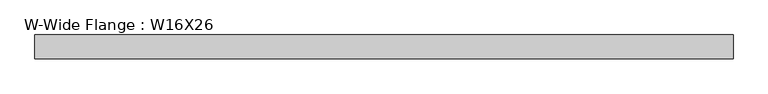
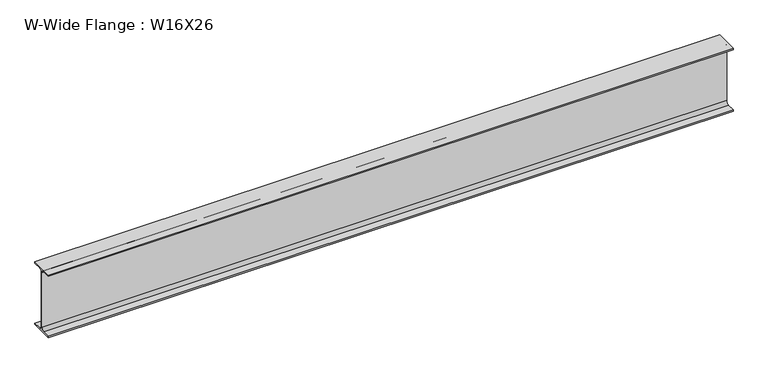
"""IFC4 building model written with IfcOpenShell, lengths in millimetres: beam geometry, W-Wide Flange : W16X26."""

from ifc_helpers import new_model, si_unit, point, frame, frame_2d, origin, place, context, project, spatial, polyline, circle_curve, trimmed, segment, composite_curve, outline, extrude, source, transform, mapped, element, save


def w_wide_flange_w16x26_55ea5116(model_context):
    return source(origin(), model_context, "Body", "SweptSolid", [
        extrude(outline(composite_curve([segment(polyline([(69.85, -190.627), (69.85, -199.39), (-69.85, -199.39), (-69.85, -190.627), (-21.3995, -190.627)]), True, "CONTINUOUS"), segment(trimmed(circle_curve(frame_2d((-21.3995, -172.4025)), 18.2245), [point((-21.3995, -190.627))], [point((-3.175, -172.4025))], True, "CARTESIAN"), True, "CONTINUOUS"), segment(polyline([(-3.175, -172.4025), (-3.175, 172.4025)]), True, "CONTINUOUS"), segment(trimmed(circle_curve(frame_2d((-21.3995, 172.4025)), 18.2245), [point((-3.175, 172.4025))], [point((-21.3995, 190.627))], True, "CARTESIAN"), True, "CONTINUOUS"), segment(polyline([(-21.3995, 190.627), (-69.85, 190.627), (-69.85, 199.39), (69.85, 199.39), (69.85, 190.627), (21.3995, 190.627)]), True, "CONTINUOUS"), segment(trimmed(circle_curve(frame_2d((21.3995, 172.4025)), 18.2245), [point((21.3995, 190.627))], [point((3.175, 172.4025))], True, "CARTESIAN"), True, "CONTINUOUS"), segment(polyline([(3.175, 172.4025), (3.175, -172.4025)]), True, "CONTINUOUS"), segment(trimmed(circle_curve(frame_2d((21.3995, -172.4025)), 18.2245), [point((3.175, -172.4025))], [point((21.3995, -190.627))], True, "CARTESIAN"), True, "CONTINUOUS"), segment(polyline([(21.3995, -190.627), (69.85, -190.627)]), True, "CONTINUOUS")], self_intersect=False)), frame((-2032.0, 0.0, 0.0), z_axis=(1.0, 0.0, 0.0), x_axis=(0.0, 1.0, 0.0)), (0.0, 0.0, 1.0), 4114.8),
    ])


if __name__ == "__main__":
    model = new_model("IFC4")
    model_context = context("Model", 3, world=origin())
    ifc_project = project(units=[si_unit("LENGTHUNIT", "METRE", prefix="MILLI")], contexts=[model_context])
    site = spatial("IfcSite", under=ifc_project)
    building = spatial("IfcBuilding", under=site)
    placement = place(None, origin())
    w_wide_flange_w16x26_shape = w_wide_flange_w16x26_55ea5116(model_context)
    element("IfcBeam", 1, ObjectType="W-Wide Flange : W16X26", at=placement, inside=building, context=model_context, shape_type="MappedRepresentation", body=[
        mapped(w_wide_flange_w16x26_shape, transform((0.0, 0.0, 0.0), x_axis=(1.0, 0.0, 0.0), y_axis=(0.0, 1.0, 0.0), z_axis=(0.0, 0.0, 1.0))),
    ])
    save(model, "model.ifc")

# Revit data of these elements
# Type "W-Wide Flange : W16X26"
#   Assembly Code = "B10"
#   W = 26
#   Length [instance default] = 5' - 0"
#   bf = 0' - 5 1/2"
#   d = 1' - 3.7"
#   k = 0' - 1 1/16"
#   k2 = 0' - 0.7175"
#   tf = 0' - 0.345"
#   tw = 0' - 0 1/4"
#   A = 0.0533333 SF
#   Structural Material [instance default] = Steel ASTM A992
# Element 1 (IfcBeam, "W-Wide Flange : W16X26")
#   Materials on its faces: "Steel ASTM A992"
# Materials
#   "Steel ASTM A992": class "Metal", colour RGB 199 199 199, transparency 0, Description = "Structural steel 50ksi", Cost = 0
